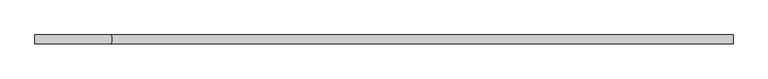
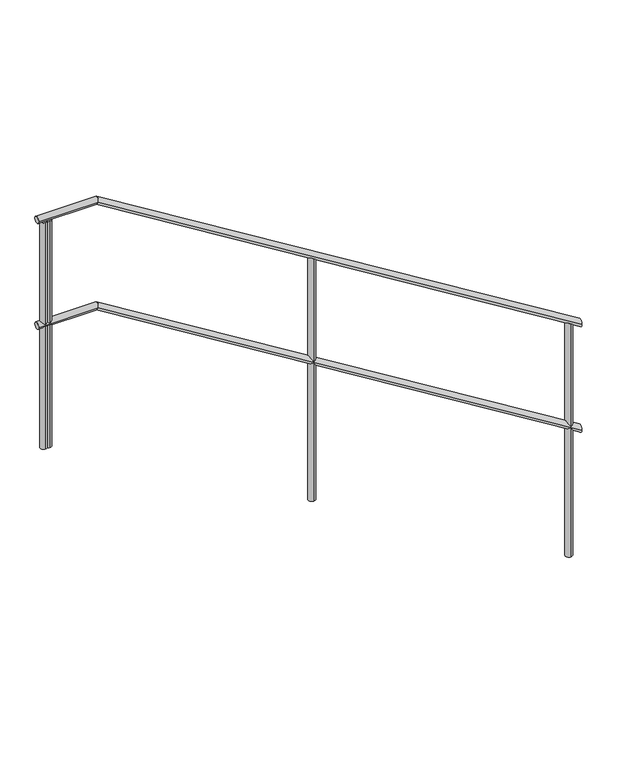
"""IFC4 building model written with IfcOpenShell, lengths in millimetres: railing geometry."""

from ifc_helpers import new_model, si_unit, point, frame, frame_2d, origin, place, context, project, spatial, circle_curve, ellipse_curve, trimmed, segment, composite_curve, outline, extrude, source, transform, mapped, element, save
from ifc_brep_helpers import plane_surface, cylinder_surface, advanced_brep


def railing_334c77da(model_context):
    return source(origin(), model_context, "Body", "SolidModel", [
        advanced_brep(
        [(68246.3017909, 72992.0208589, -450.9609787), (68246.3017909, 72962.0208589, -450.9609787), (66082.0450053, 72992.0208589, 885.0), (66082.0450053, 72962.0208589, 885.0), (65816.3017909, 72992.0208589, 885.0), (65816.3017909, 72962.0208589, 885.0)],
        [
            (0, 1, ellipse_curve(frame((68246.3017909, 72977.0208589, -450.9609787), z_axis=(1.0, 0.0, 0.0), x_axis=(0.0, 0.0, -1.0)), 17.6276454, 15.0)),
            (1, 0, ellipse_curve(frame((68246.3017909, 72977.0208589, -450.9609787), z_axis=(1.0, 0.0, 0.0), x_axis=(0.0, 0.0, -1.0)), 17.6276454, 15.0)),
            (0, 2),
            (2, 3, ellipse_curve(frame((66082.0450053, 72977.0208589, 885.0), z_axis=(0.9620125025549409, 0.0, -0.27300539358770864), x_axis=(-0.27300539358770803, 0.0, -0.9620125025549412)), 15.5923129, 15.0)),
            (3, 1),
            (3, 2, ellipse_curve(frame((66082.0450053, 72977.0208589, 885.0), z_axis=(0.9620125025549409, 0.0, -0.27300539358770864), x_axis=(-0.27300539358770803, 0.0, -0.9620125025549412)), 15.5923129, 15.0)),
            (4, 5, circle_curve(frame((65816.3017909, 72977.0208589, 885.0), z_axis=(-1.0, 0.0, 0.0), x_axis=(0.0, -1.0, 0.0)), 15.0)),
            (5, 4, circle_curve(frame((65816.3017909, 72977.0208589, 885.0), z_axis=(-1.0, 0.0, 0.0), x_axis=(0.0, -1.0, 0.0)), 15.0)),
            (2, 4),
            (5, 3),
        ],
        [
            plane_surface(frame((68246.3017909, 72977.0208589, -433.3333333), z_axis=(1.0, 0.0, 0.0), x_axis=(0.0, -1.0, 0.0))),
            cylinder_surface(frame((68238.4227528, 72977.0208589, -446.097375), z_axis=(0.8509361101440404, 0.0, -0.5252692037926168), x_axis=(0.0, -1.0, 0.0)), 15.0),
            plane_surface(frame((65816.3017909, 72977.0208589, 900.0), z_axis=(-1.0, 0.0, 0.0), x_axis=(0.0, -1.0, 0.0))),
            cylinder_surface(frame((66086.3017909, 72977.0208589, 885.0), z_axis=(1.0, 0.0, 0.0), x_axis=(0.0, -1.0, 0.0)), 15.0),
        ],
        [
            (0, [[1, 2]]),
            (1, [[-1, 3, 4, 5]]),
            (1, [[-2, -5, 6, -3]]),
            (2, [[7, 8]]),
            (3, [[-4, 9, -8, 10]]),
            (3, [[-6, -10, -7, -9]]),
        ],
    ),
        advanced_brep(
        [(68246.3017909, 72992.0208589, 49.0390213), (68246.3017909, 72962.0208589, 49.0390213), (66082.0450053, 72992.0208589, 1385.0), (66082.0450053, 72962.0208589, 1385.0), (65816.3017909, 72992.0208589, 1385.0), (65816.3017909, 72962.0208589, 1385.0)],
        [
            (0, 1, ellipse_curve(frame((68246.3017909, 72977.0208589, 49.0390213), z_axis=(1.0, 0.0, 0.0), x_axis=(0.0, 0.0, -1.0)), 17.6276454, 15.0)),
            (1, 0, ellipse_curve(frame((68246.3017909, 72977.0208589, 49.0390213), z_axis=(1.0, 0.0, 0.0), x_axis=(0.0, 0.0, -1.0)), 17.6276454, 15.0)),
            (0, 2),
            (2, 3, ellipse_curve(frame((66082.0450053, 72977.0208589, 1385.0), z_axis=(0.9620125025549409, 0.0, -0.27300539358770864), x_axis=(-0.27300539358770803, 0.0, -0.9620125025549412)), 15.5923129, 15.0)),
            (3, 1),
            (3, 2, ellipse_curve(frame((66082.0450053, 72977.0208589, 1385.0), z_axis=(0.9620125025549409, 0.0, -0.27300539358770864), x_axis=(-0.27300539358770803, 0.0, -0.9620125025549412)), 15.5923129, 15.0)),
            (4, 5, circle_curve(frame((65816.3017909, 72977.0208589, 1385.0), z_axis=(-1.0, 0.0, 0.0), x_axis=(0.0, -1.0, 0.0)), 15.0)),
            (5, 4, circle_curve(frame((65816.3017909, 72977.0208589, 1385.0), z_axis=(-1.0, 0.0, 0.0), x_axis=(0.0, -1.0, 0.0)), 15.0)),
            (2, 4),
            (5, 3),
        ],
        [
            plane_surface(frame((68246.3017909, 72977.0208589, 66.6666667), z_axis=(1.0, 0.0, 0.0), x_axis=(0.0, -1.0, 0.0))),
            cylinder_surface(frame((68238.4227528, 72977.0208589, 53.902625), z_axis=(0.8509361101440404, 0.0, -0.5252692037926168), x_axis=(0.0, -1.0, 0.0)), 15.0),
            plane_surface(frame((65816.3017909, 72977.0208589, 1400.0), z_axis=(-1.0, 0.0, 0.0), x_axis=(0.0, -1.0, 0.0))),
            cylinder_surface(frame((66086.3017909, 72977.0208589, 1385.0), z_axis=(1.0, 0.0, 0.0), x_axis=(0.0, -1.0, 0.0)), 15.0),
        ],
        [
            (0, [[1, 2]]),
            (1, [[-1, 3, 4, 5]]),
            (1, [[-2, -5, 6, -3]]),
            (2, [[7, 8]]),
            (3, [[-4, 9, -8, 10]]),
            (3, [[-6, -10, -7, -9]]),
        ],
    ),
        extrude(outline(composite_curve([segment(trimmed(circle_curve(frame_2d((65846.3017909, 72977.0208589)), 15.0), [point((65846.3017909, 72992.0208589))], [point((65846.3017909, 72962.0208589))], False, "CARTESIAN"), True, "CONTINUOUS"), segment(trimmed(circle_curve(frame_2d((65846.3017909, 72977.0208589)), 15.0), [point((65846.3017909, 72962.0208589))], [point((65846.3017909, 72992.0208589))], False, "CARTESIAN"), True, "CONTINUOUS")], self_intersect=False)), frame((0.0, 0.0, 300.0), z_axis=(0.0, 0.0, 1.0), x_axis=(1.0, 0.0, 0.0)), (0.0, 0.0, 1.0), 1070.0),
        advanced_brep(
        [(67046.3017909, 72962.0208589, 777.4074074), (67046.3017909, 72992.0208589, 777.4074074), (67046.3017909, 72992.0208589, -366.6666667), (67046.3017909, 72962.0208589, -366.6666667)],
        [
            (0, 1, ellipse_curve(frame((67046.3017909, 72977.0208589, 777.4074074), z_axis=(-0.5252692037926167, 0.0, -0.8509361101440406), x_axis=(-0.8509361101440406, 0.0, 0.5252692037926162)), 17.6276454, 15.0)),
            (1, 2),
            (2, 3, circle_curve(frame((67046.3017909, 72977.0208589, -366.6666667), z_axis=(0.0, 0.0, 1.0), x_axis=(0.0, 1.0, 0.0)), 15.0)),
            (3, 0),
            (3, 2, circle_curve(frame((67046.3017909, 72977.0208589, -366.6666667), z_axis=(0.0, 0.0, 1.0), x_axis=(0.0, 1.0, 0.0)), 15.0)),
            (1, 0, ellipse_curve(frame((67046.3017909, 72977.0208589, 777.4074074), z_axis=(-0.5252692037926167, 0.0, -0.8509361101440406), x_axis=(-0.8509361101440406, 0.0, 0.5252692037926162)), 17.6276454, 15.0)),
        ],
        [
            cylinder_surface(frame((67046.3017909, 72977.0208589, -466.6666667), z_axis=(0.0, 0.0, 1.0), x_axis=(0.0, 1.0, 0.0)), 15.0),
            plane_surface(frame((67021.3017909, 73002.0208589, 792.8395062), z_axis=(0.5252692037926167, 0.0, 0.8509361101440406), x_axis=(0.0, -1.0, 0.0))),
            plane_surface(frame((67071.3017909, 73002.0208589, -366.6666667), z_axis=(0.0, 0.0, -1.0), x_axis=(0.0, -1.0, 0.0))),
        ],
        [
            (0, [[1, 2, 3, 4]]),
            (0, [[5, -2, 6, -4]]),
            (1, [[-6, -1]]),
            (2, [[-5, -3]]),
        ],
    ),
        extrude(outline(composite_curve([segment(trimmed(circle_curve(frame_2d((65866.3017909, 72977.0208589)), 15.0), [point((65866.3017909, 72992.0208589))], [point((65866.3017909, 72962.0208589))], False, "CARTESIAN"), True, "CONTINUOUS"), segment(trimmed(circle_curve(frame_2d((65866.3017909, 72977.0208589)), 15.0), [point((65866.3017909, 72962.0208589))], [point((65866.3017909, 72992.0208589))], False, "CARTESIAN"), True, "CONTINUOUS")], self_intersect=False)), frame((0.0, 0.0, 300.0), z_axis=(0.0, 0.0, 1.0), x_axis=(1.0, 0.0, 0.0)), (0.0, 0.0, 1.0), 1070.0),
        advanced_brep(
        [(68196.3017909, 72962.0208589, 67.5308642), (68196.3017909, 72992.0208589, 67.5308642), (68196.3017909, 72992.0208589, -1033.3333333), (68196.3017909, 72962.0208589, -1033.3333333)],
        [
            (0, 1, ellipse_curve(frame((68196.3017909, 72977.0208589, 67.5308642), z_axis=(-0.5252692037926167, 0.0, -0.8509361101440406), x_axis=(-0.8509361101440406, 0.0, 0.5252692037926162)), 17.6276454, 15.0)),
            (1, 2),
            (2, 3, circle_curve(frame((68196.3017909, 72977.0208589, -1033.3333333), z_axis=(0.0, 0.0, 1.0), x_axis=(0.0, 1.0, 0.0)), 15.0)),
            (3, 0),
            (3, 2, circle_curve(frame((68196.3017909, 72977.0208589, -1033.3333333), z_axis=(0.0, 0.0, 1.0), x_axis=(0.0, 1.0, 0.0)), 15.0)),
            (1, 0, ellipse_curve(frame((68196.3017909, 72977.0208589, 67.5308642), z_axis=(-0.5252692037926167, 0.0, -0.8509361101440406), x_axis=(-0.8509361101440406, 0.0, 0.5252692037926162)), 17.6276454, 15.0)),
        ],
        [
            cylinder_surface(frame((68196.3017909, 72977.0208589, -1133.3333333), z_axis=(0.0, 0.0, 1.0), x_axis=(0.0, 1.0, 0.0)), 15.0),
            plane_surface(frame((68171.3017909, 73002.0208589, 82.962963), z_axis=(0.5252692037926167, 0.0, 0.8509361101440406), x_axis=(0.0, -1.0, 0.0))),
            plane_surface(frame((68221.3017909, 73002.0208589, -1033.3333333), z_axis=(0.0, 0.0, -1.0), x_axis=(0.0, -1.0, 0.0))),
        ],
        [
            (0, [[1, 2, 3, 4]]),
            (0, [[5, -2, 6, -4]]),
            (1, [[-6, -1]]),
            (2, [[-5, -3]]),
        ],
    ),
    ])


if __name__ == "__main__":
    model = new_model("IFC4")
    model_context = context("Model", 3, world=origin())
    ifc_project = project(units=[si_unit("LENGTHUNIT", "METRE", prefix="MILLI")], contexts=[model_context])
    site = spatial("IfcSite", under=ifc_project)
    building = spatial("IfcBuilding", under=site)
    placement = place(None, origin())
    railing_shape = railing_334c77da(model_context)
    element("IfcRailing", 1, at=placement, inside=building, context=model_context, shape_type="MappedRepresentation", body=[
        mapped(railing_shape, transform((0.0, 0.0, 0.0), x_axis=(1.0, 0.0, 0.0), y_axis=(0.0, 1.0, 0.0), z_axis=(0.0, 0.0, 1.0))),
    ])
    save(model, "model.ifc")
